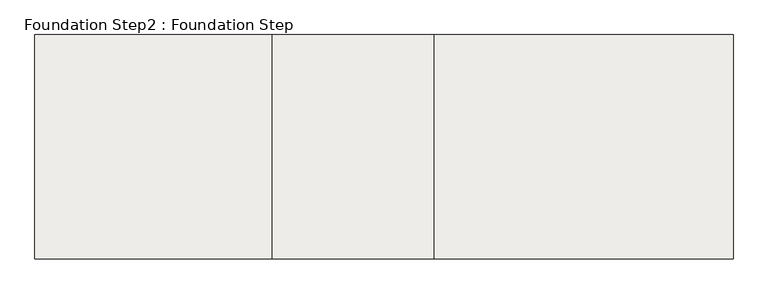
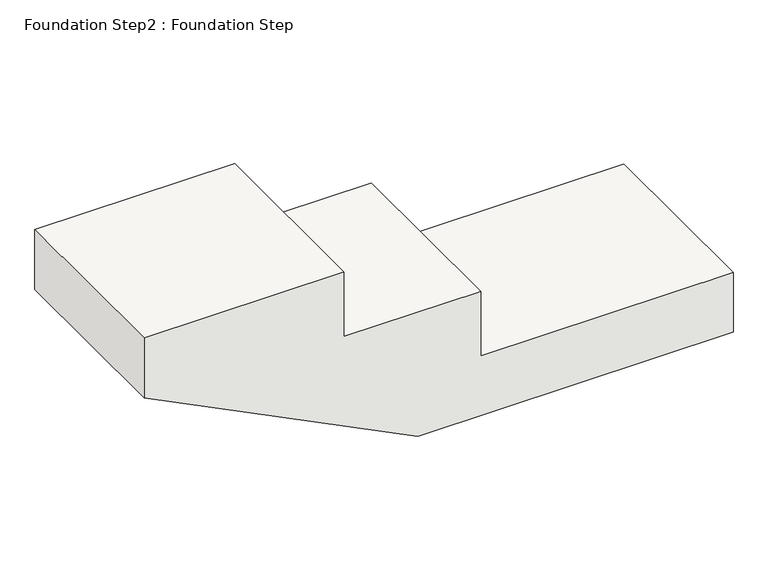
"""IFC4 building model written with IfcOpenShell, lengths in millimetres: slab geometry, Foundation Step2 : Foundation Step."""

from ifc_helpers import new_model, si_unit, frame, origin, place, context, project, spatial, polyline, outline, extrude, source, transform, mapped, element, save


def foundation_step2_foundation_step_839b83da(model_context):
    return source(origin(), model_context, "Body", "SweptSolid", [
        extrude(outline(polyline([(-1092.2, -46445.5350821), (-1092.2, -47410.7350821), (-1397.0, -47410.7350821), (-2057.4, -46089.9350821), (-2057.4, -44565.9350821), (-1752.6, -44565.9350821), (-1752.6, -45785.1350821), (-1422.4, -45785.1350821), (-1422.4, -46445.5350821), (-1092.2, -46445.5350821)])), frame((0.0, 12628.3018471, 0.0), z_axis=(0.0, 1.0, 0.0), x_axis=(0.0, 0.0, 1.0)), (0.0, 0.0, 1.0), 914.4),
    ])


if __name__ == "__main__":
    model = new_model("IFC4")
    model_context = context("Model", 3, world=origin())
    ifc_project = project(units=[si_unit("LENGTHUNIT", "METRE", prefix="MILLI")], contexts=[model_context])
    site = spatial("IfcSite", under=ifc_project)
    building = spatial("IfcBuilding", under=site)
    placement = place(None, origin())
    foundation_step2_foundation_step_shape = foundation_step2_foundation_step_839b83da(model_context)
    element("IfcSlab", 1, ObjectType="Foundation Step2 : Foundation Step", at=placement, inside=building, context=model_context, shape_type="MappedRepresentation", body=[
        mapped(foundation_step2_foundation_step_shape, transform((0.0, 0.0, 0.0), x_axis=(1.0, 0.0, 0.0), y_axis=(0.0, 1.0, 0.0), z_axis=(0.0, 0.0, 1.0))),
    ])
    save(model, "model.ifc")

# Revit data of these elements
# Type "Foundation Step2 : Foundation Step"
#   Structural Material = Concrete, Cast-in-Place gray
# Materials
#   "Concrete, Cast-in-Place gray": class "Concrete", colour RGB 192 192 192, transparency 0, Description = "Cast-in-place concrete", Cost = 0
